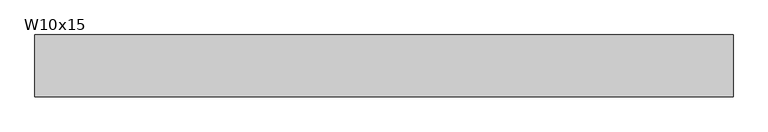
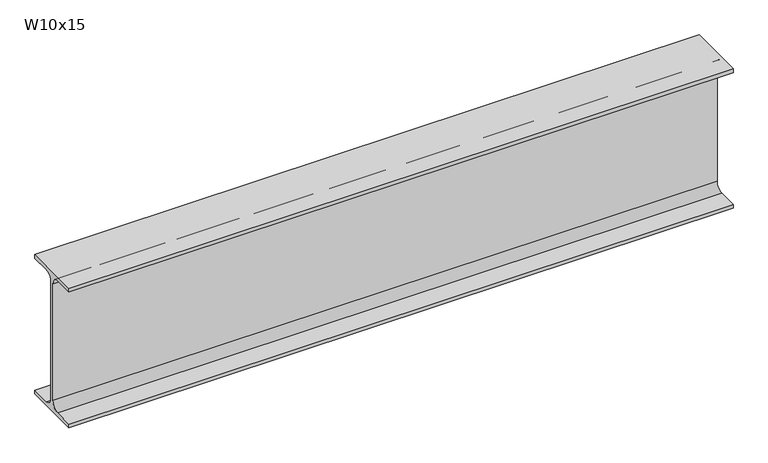
"""IFC4 building model written with IfcOpenShell, lengths in millimetres: beam geometry, RME W-Wide Flange : W10x15."""

from ifc_helpers import new_model, si_unit, point, frame, frame_2d, origin, place, context, project, spatial, polyline, circle_curve, trimmed, segment, composite_curve, outline, extrude, source, transform, mapped, element, save


def w10x15_48f5b6d0(model_context):
    return source(origin(), model_context, "Body", "SweptSolid", [
        extrude(outline(composite_curve([segment(polyline([(50.8, -120.142), (50.8, -127.0), (-50.8, -127.0), (-50.8, -120.142), (-16.7005, -120.142)]), True, "CONTINUOUS"), segment(trimmed(circle_curve(frame_2d((-16.7005, -106.3625)), 13.7795), [point((-16.7005, -120.142))], [point((-2.921, -106.3625))], True, "CARTESIAN"), True, "CONTINUOUS"), segment(polyline([(-2.921, -106.3625), (-2.921, 106.3625)]), True, "CONTINUOUS"), segment(trimmed(circle_curve(frame_2d((-16.7005, 106.3625)), 13.7795), [point((-2.921, 106.3625))], [point((-16.7005, 120.142))], True, "CARTESIAN"), True, "CONTINUOUS"), segment(polyline([(-16.7005, 120.142), (-50.8, 120.142), (-50.8, 127.0), (50.8, 127.0), (50.8, 120.142), (16.7005, 120.142)]), True, "CONTINUOUS"), segment(trimmed(circle_curve(frame_2d((16.7005, 106.3625)), 13.7795), [point((16.7005, 120.142))], [point((2.921, 106.3625))], True, "CARTESIAN"), True, "CONTINUOUS"), segment(polyline([(2.921, 106.3625), (2.921, -106.3625)]), True, "CONTINUOUS"), segment(trimmed(circle_curve(frame_2d((16.7005, -106.3625)), 13.7795), [point((2.921, -106.3625))], [point((16.7005, -120.142))], True, "CARTESIAN"), True, "CONTINUOUS"), segment(polyline([(16.7005, -120.142), (50.8, -120.142)]), True, "CONTINUOUS")], self_intersect=False)), frame((-584.2, 0.0, 0.0), z_axis=(1.0, 0.0, 0.0), x_axis=(0.0, 1.0, 0.0)), (0.0, 0.0, 1.0), 1142.9999994),
    ])


if __name__ == "__main__":
    model = new_model("IFC4")
    model_context = context("Model", 3, world=origin())
    ifc_project = project(units=[si_unit("LENGTHUNIT", "METRE", prefix="MILLI")], contexts=[model_context])
    site = spatial("IfcSite", under=ifc_project)
    building = spatial("IfcBuilding", under=site)
    placement = place(None, origin())
    w10x15_shape = w10x15_48f5b6d0(model_context)
    element("IfcBeam", 1, ObjectType="RME W-Wide Flange : W10x15", at=placement, inside=building, context=model_context, shape_type="MappedRepresentation", body=[
        mapped(w10x15_shape, transform((0.0, 0.0, 0.0), x_axis=(1.0, 0.0, 0.0), y_axis=(0.0, 1.0, 0.0), z_axis=(0.0, 0.0, 1.0))),
    ])
    save(model, "model.ifc")

# Revit data of these elements
# Type "RME W-Wide Flange : W10x15"
#   WELD P [instance default] = ""
#   WELD LE [instance default] = ""
#   WELD D [instance default] = ""
#   TOP SECTION SIZE [instance default] = ""
#   TOP SECTION LENGTH [instance default] = ""
#   REMARKS [instance default] = ""
#   REINF TYPE [instance default] = ""
#   Nominal Size = "W24"
#   End Bearing Capacity [instance default] = ""
#   BOT SECTION SIZE [instance default] = ""
#   BOT SECTION LENGTH [instance default] = ""
#   Assembly Code = "B10"
#   W = 15
#   Start Extension Calculation [instance default] = 10' - 0"
#   Start Extension [instance default] = -0' - 0 1/2"
#   End Extension Calculation [instance default] = 10' - 0"
#   End Extension [instance default] = -0' - 0 1/2"
#   Length [instance default] = 5' - 0"
#   bf = 0' - 4"
#   d = 0' - 10"
#   k = 0' - 0 13/16"
#   k2 = 0' - 0.5425"
#   tf = 0' - 0.27"
#   tw = 0' - 0.23"
#   A = 0.030625 SF
#   Structural Material [instance default] = Metal - Steel - ASTM A992
# Element 1 (IfcBeam, "RME W-Wide Flange : W10x15")
#   Length = 3' - 9"
#   Materials on its faces: "Metal - Steel - ASTM A992"
# Materials
#   "Metal - Steel - ASTM A992": class "Metal", colour RGB 255 128 0, transparency 0
